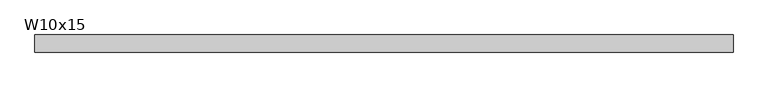
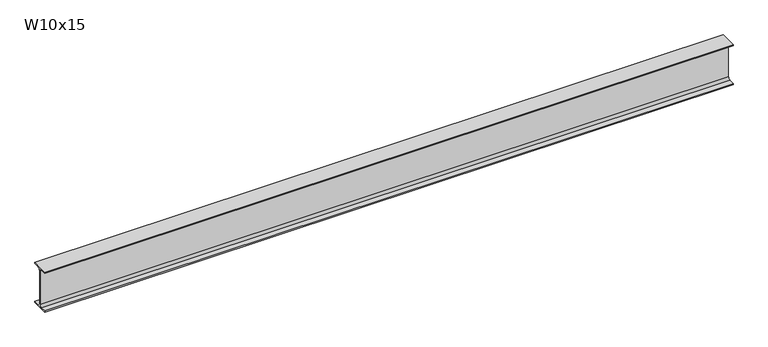
"""IFC4 building model written with IfcOpenShell, lengths in millimetres: beam geometry, RME W-Wide Flange : W10x15."""

from ifc_helpers import new_model, si_unit, point, frame, frame_2d, origin, place, context, project, spatial, polyline, circle_curve, trimmed, segment, composite_curve, outline, extrude, source, transform, mapped, element, save


def w10x15_c3b9fcee(model_context):
    return source(origin(), model_context, "Body", "SweptSolid", [
        extrude(outline(composite_curve([segment(polyline([(50.8, -120.142), (50.8, -127.0), (-50.8, -127.0), (-50.8, -120.142), (-16.7005, -120.142)]), True, "CONTINUOUS"), segment(trimmed(circle_curve(frame_2d((-16.7005, -106.3625)), 13.7795), [point((-16.7005, -120.142))], [point((-2.921, -106.3625))], True, "CARTESIAN"), True, "CONTINUOUS"), segment(polyline([(-2.921, -106.3625), (-2.921, 106.3625)]), True, "CONTINUOUS"), segment(trimmed(circle_curve(frame_2d((-16.7005, 106.3625)), 13.7795), [point((-2.921, 106.3625))], [point((-16.7005, 120.142))], True, "CARTESIAN"), True, "CONTINUOUS"), segment(polyline([(-16.7005, 120.142), (-50.8, 120.142), (-50.8, 127.0), (50.8, 127.0), (50.8, 120.142), (16.7005, 120.142)]), True, "CONTINUOUS"), segment(trimmed(circle_curve(frame_2d((16.7005, 106.3625)), 13.7795), [point((16.7005, 120.142))], [point((2.921, 106.3625))], True, "CARTESIAN"), True, "CONTINUOUS"), segment(polyline([(2.921, 106.3625), (2.921, -106.3625)]), True, "CONTINUOUS"), segment(trimmed(circle_curve(frame_2d((16.7005, -106.3625)), 13.7795), [point((2.921, -106.3625))], [point((16.7005, -120.142))], True, "CARTESIAN"), True, "CONTINUOUS"), segment(polyline([(16.7005, -120.142), (50.8, -120.142)]), True, "CONTINUOUS")], self_intersect=False)), frame((-2074.646432, 0.0, 0.0), z_axis=(1.0, 0.0, 0.0), x_axis=(0.0, 1.0, 0.0)), (0.0, 0.0, 1.0), 4136.5928633),
    ])


if __name__ == "__main__":
    model = new_model("IFC4")
    model_context = context("Model", 3, world=origin())
    ifc_project = project(units=[si_unit("LENGTHUNIT", "METRE", prefix="MILLI")], contexts=[model_context])
    site = spatial("IfcSite", under=ifc_project)
    building = spatial("IfcBuilding", under=site)
    placement = place(None, origin())
    w10x15_shape = w10x15_c3b9fcee(model_context)
    element("IfcBeam", 1, ObjectType="RME W-Wide Flange : W10x15", at=placement, inside=building, context=model_context, shape_type="MappedRepresentation", body=[
        mapped(w10x15_shape, transform((0.0, 0.0, 0.0), x_axis=(1.0, 0.0, 0.0), y_axis=(0.0, 1.0, 0.0), z_axis=(0.0, 0.0, 1.0))),
    ])
    save(model, "model.ifc")

# Revit data of these elements
# Type "RME W-Wide Flange : W10x15"
#   WELD P [instance default] = ""
#   WELD LE [instance default] = ""
#   WELD D [instance default] = ""
#   TOP SECTION SIZE [instance default] = ""
#   TOP SECTION LENGTH [instance default] = ""
#   REMARKS [instance default] = ""
#   REINF TYPE [instance default] = ""
#   Nominal Size = "W24"
#   End Bearing Capacity [instance default] = ""
#   BOT SECTION SIZE [instance default] = ""
#   BOT SECTION LENGTH [instance default] = ""
#   Assembly Code = "B10"
#   W = 15
#   Start Extension Calculation [instance default] = 10' - 0"
#   Start Extension [instance default] = -0' - 0 1/2"
#   End Extension Calculation [instance default] = 10' - 0"
#   End Extension [instance default] = -0' - 0 1/2"
#   Length [instance default] = 5' - 0"
#   bf = 0' - 4"
#   d = 0' - 10"
#   k = 0' - 0 13/16"
#   k2 = 0' - 0.5425"
#   tf = 0' - 0.27"
#   tw = 0' - 0.23"
#   A = 0.030625 SF
#   Structural Material [instance default] = Metal - Steel - ASTM A992
# Element 1 (IfcBeam, "RME W-Wide Flange : W10x15")
#   Length = 13' - 7.35799"
#   Materials on its faces: "Metal - Steel - ASTM A992"
# Materials
#   "Metal - Steel - ASTM A992": class "Metal", colour RGB 255 128 0, transparency 0
